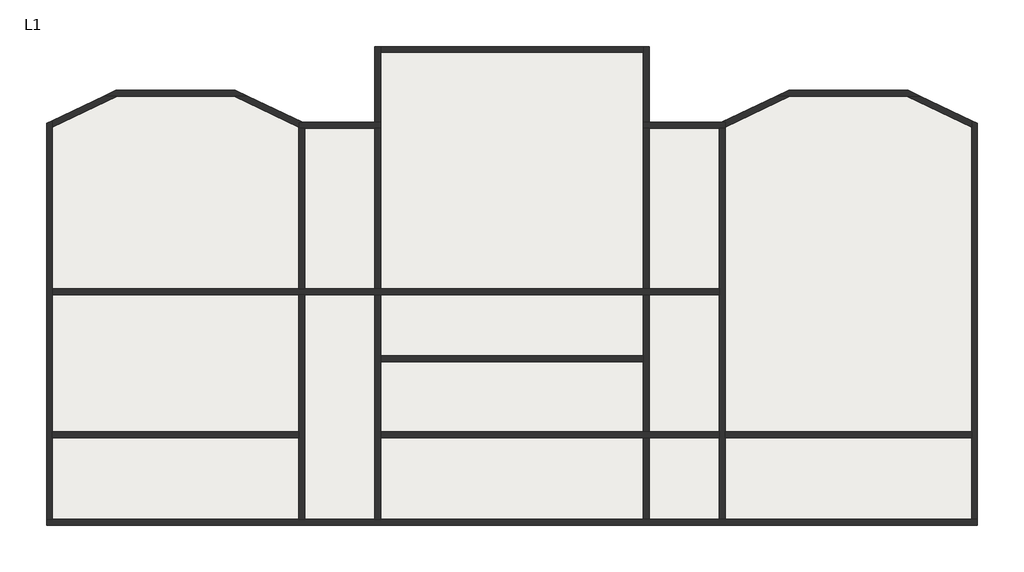
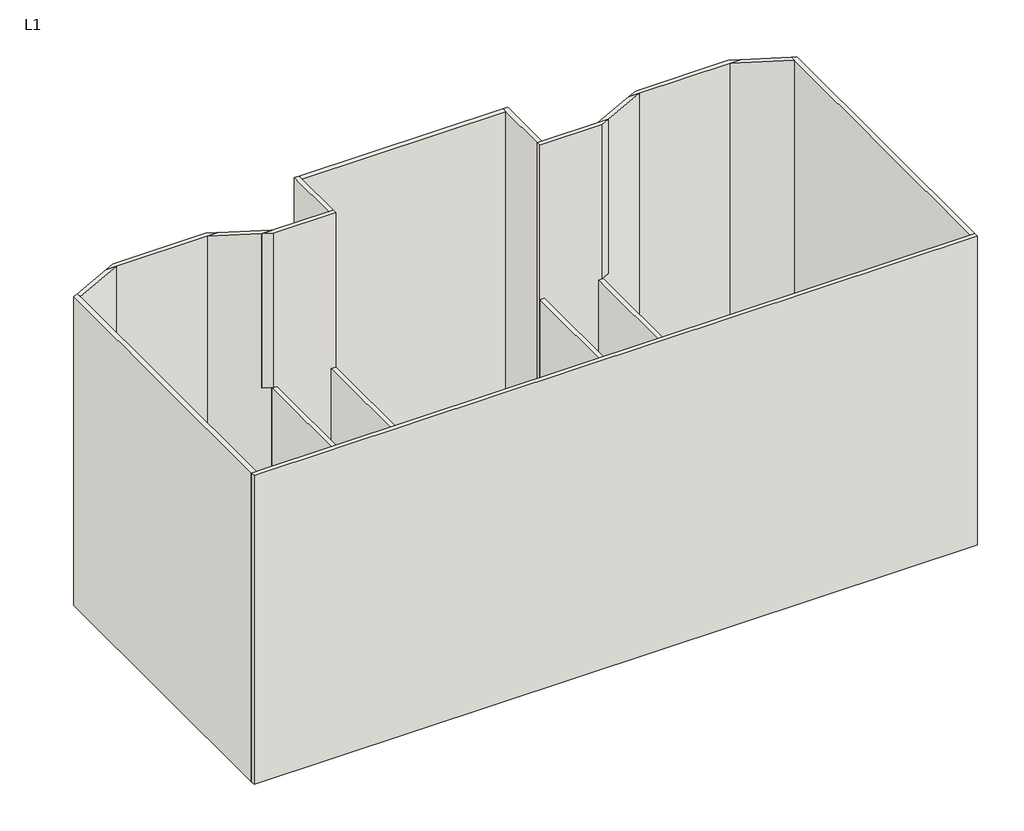
# One storey: 22 walls, 1 slab.
"""IFC4 building model written with IfcOpenShell, lengths in millimetres."""

import ifcopenshell
import ifcopenshell.guid

model = None  # the IFC model being written
_history = None  # IfcOwnerHistory: only IFC2X3 demands one
_inside = {}  # id of a spatial element -> (the spatial element, [elements in it])
_under = {}  # id of a project, library or spatial element -> (it, [spatial elements below it])
_declared = {}  # id of a project -> (the project, [libraries it declares])
_typed = {}  # id of a type object -> (the type object, [elements of that type])
_made_of = {}  # id of a material, layer set ... -> (it, [elements and type objects made of it])


def new_model(schema):
    """Start an empty IFC model of exactly this schema.

    Asked for "IFC4X3", IfcOpenShell would pick the latest addendum, in which some entities
    have other attributes; the version numbers below select the first issue.
    IFC2X3 requires an IfcOwnerHistory on every rooted entity: one is made here for all.
    """
    global model, _history
    if schema == "IFC4X3":
        model = ifcopenshell.file(schema_version=(4, 3, 0, 0))
    else:
        model = ifcopenshell.file(schema=schema)
    _inside.clear()
    _under.clear()
    _declared.clear()
    _typed.clear()
    _made_of.clear()
    _history = None
    if model.schema == "IFC2X3":
        org = make("IfcOrganization", Name="unknown")
        user = make(
            "IfcPersonAndOrganization",
            ThePerson=make("IfcPerson", FamilyName="unknown"),
            TheOrganization=org,
        )
        app = make(
            "IfcApplication",
            ApplicationDeveloper=org,
            Version="unknown",
            ApplicationFullName="unknown",
            ApplicationIdentifier="unknown",
        )
        _history = make(
            "IfcOwnerHistory",
            OwningUser=user,
            OwningApplication=app,
            ChangeAction="ADDED",
            CreationDate=0,
        )
    return model


def make(cls, **values):
    """One entity of the class cls with the attributes given. An attribute that is None is left unset."""
    return model.create_entity(
        cls, **{name: value for name, value in values.items() if value is not None}
    )


def rooted(cls, **values):
    """An entity with a GlobalId (a new one), such as an element, a storey or a relation."""
    return make(cls, GlobalId=ifcopenshell.guid.new(), OwnerHistory=_history, **values)


def si_unit(unit_type, name, prefix=None):
    """IfcSIUnit, for example si_unit("LENGTHUNIT", "METRE", prefix="MILLI")."""
    return make("IfcSIUnit", UnitType=unit_type, Prefix=prefix, Name=name)


def assignment(units):
    """IfcUnitAssignment: the units of a project."""
    return None if units is None else make("IfcUnitAssignment", Units=units)


def point(xyz):
    """IfcCartesianPoint."""
    return None if xyz is None else make("IfcCartesianPoint", Coordinates=xyz)


def direction(xyz):
    """IfcDirection."""
    return None if xyz is None else make("IfcDirection", DirectionRatios=xyz)


def frame(location, z_axis=None, x_axis=None):
    """IfcAxis2Placement3D, a coordinate frame: its origin and axes. An axis left out is left unset."""
    return make(
        "IfcAxis2Placement3D",
        Location=point(location),
        Axis=direction(z_axis),
        RefDirection=direction(x_axis),
    )


def origin():
    """The frame at (0, 0, 0) with its axes left unset."""
    return frame((0.0, 0.0, 0.0))


def origin_with_axes():
    """The frame at (0, 0, 0) with the z axis (0, 0, 1) and the x axis (1, 0, 0) written out."""
    return frame((0.0, 0.0, 0.0), z_axis=(0.0, 0.0, 1.0), x_axis=(1.0, 0.0, 0.0))


def place(relative_to, where):
    """IfcLocalPlacement: puts the frame where relative to a parent placement (None: the world)."""
    return make(
        "IfcLocalPlacement", PlacementRelTo=relative_to, RelativePlacement=where
    )


def context(
    kind, dimensions, precision=None, world=None, true_north=None, identifier=None
):
    """IfcGeometricRepresentationContext, for example the 3D "Model" context."""
    return make(
        "IfcGeometricRepresentationContext",
        ContextIdentifier=identifier,
        ContextType=kind,
        CoordinateSpaceDimension=dimensions,
        Precision=precision,
        WorldCoordinateSystem=world,
        TrueNorth=true_north,
    )


def project(units=None, contexts=None):
    """IfcProject with its units and contexts."""
    return rooted(
        "IfcProject",
        Name="project",
        RepresentationContexts=contexts,
        UnitsInContext=assignment(units),
    )


def spatial(cls, under=None, at=None, **own):
    """A site, building, storey or space (cls), placed at a placement, below another one or the project."""
    s = rooted(cls, ObjectPlacement=at, **own)
    if under is not None:
        _under.setdefault(under.id(), (under, []))[1].append(s)
    return s


def polyline(points):
    """IfcPolyline through the points."""
    return make("IfcPolyline", Points=[point(p) for p in points])


def outline(outer, holes=None, kind="AREA"):
    """IfcArbitraryClosedProfileDef: a profile drawn as a closed curve; with holes, ...WithVoids."""
    if holes is None:
        return make("IfcArbitraryClosedProfileDef", ProfileType=kind, OuterCurve=outer)
    return make(
        "IfcArbitraryProfileDefWithVoids",
        ProfileType=kind,
        OuterCurve=outer,
        InnerCurves=holes,
    )


def extrude(swept, where, along, depth):
    """IfcExtrudedAreaSolid: the profile swept, set in the frame where, extruded along a direction by depth."""
    return make(
        "IfcExtrudedAreaSolid",
        SweptArea=swept,
        Position=where,
        ExtrudedDirection=direction(along),
        Depth=depth,
    )


def faces_of(points, faces, orient=None, outer=None):
    """IfcFace entities. A face is a list of loops; a loop is a list of indices into points, from 0.

    orient and outer hold one flag for each loop. By default every Orientation is true, the
    first loop of a face is its IfcFaceOuterBound and the others are IfcFaceBound.
    """
    made = []
    for i, loops in enumerate(faces):
        bounds = []
        for j, loop in enumerate(loops):
            is_outer = j == 0 if outer is None else outer[i][j]
            bounds.append(
                make(
                    "IfcFaceOuterBound" if is_outer else "IfcFaceBound",
                    Bound=make("IfcPolyLoop", Polygon=[points[k] for k in loop]),
                    Orientation=True if orient is None else orient[i][j],
                )
            )
        made.append(make("IfcFace", Bounds=bounds))
    return made


def faceted_brep(points, faces, orient=None, outer=None, voids=None):
    """IfcFacetedBrep: a solid bounded by flat faces; with voids (closed shells), ...WithVoids."""
    shared = [point(p) for p in points]
    hull = make("IfcClosedShell", CfsFaces=faces_of(shared, faces, orient, outer))
    if voids is None:
        return make("IfcFacetedBrep", Outer=hull)
    return make(
        "IfcFacetedBrepWithVoids",
        Outer=hull,
        Voids=[
            make(cls, CfsFaces=faces_of(shared, fs, o, b)) for cls, fs, o, b in voids
        ],
    )


def shape(context_of_items, identifier, shape_type, items):
    """IfcShapeRepresentation: the items that make up one representation, for example the "Body"."""
    return make(
        "IfcShapeRepresentation",
        ContextOfItems=context_of_items,
        RepresentationIdentifier=identifier,
        RepresentationType=shape_type,
        Items=items,
    )


def made_of(thing, what):
    """Note that an element or type object is made of a material, layer set ...; save() writes the relation."""
    if what is not None:
        _made_of.setdefault(what.id(), (what, []))[1].append(thing)
    return thing


def element(
    cls,
    number,
    at=None,
    inside=None,
    cuts=None,
    type_object=None,
    material=None,
    context=None,
    identifier="Body",
    shape_type=None,
    held_by="IfcProductDefinitionShape",
    body=None,
    shapes=None,
    **own,
):
    """One element of the class cls, such as IfcWall. Its Tag is "e" and its number.

    at: its placement. inside: the storey or other place that contains it. cuts: it is an
    opening in that element (IfcRelVoidsElement). A single representation is given by context,
    identifier, shape_type and body (its items); several are given by shapes. held_by: the class
    of the entity that holds the representations. save() writes the other relations.
    """
    e = rooted(cls, Tag="e%d" % number, ObjectPlacement=at, **own)
    if body is not None:
        shapes = [shape(context, identifier, shape_type, body)]
    if shapes is not None:
        e.Representation = make(held_by, Representations=shapes)
    if inside is not None:
        _inside.setdefault(inside.id(), (inside, []))[1].append(e)
    if cuts is not None:
        rooted(
            "IfcRelVoidsElement", RelatingBuildingElement=cuts, RelatedOpeningElement=e
        )
    if type_object is not None:
        _typed.setdefault(type_object.id(), (type_object, []))[1].append(e)
    return made_of(e, material)


def aggregate(whole, parts):
    """IfcRelAggregates: a whole, such as a stair, and the parts it consists of."""
    return rooted("IfcRelAggregates", RelatingObject=whole, RelatedObjects=parts)


def save(model, path):
    """Write the relations noted so far, then the file.

    IfcRelAggregates (storeys below a building ...), IfcRelContainedInSpatialStructure (elements
    in a storey), IfcRelDefinesByType, IfcRelAssociatesMaterial and IfcRelDeclares: one each for
    every whole, place, type object, material and project.
    """
    for whole, parts in _under.values():
        aggregate(whole, parts)
    for where, things in _inside.values():
        rooted(
            "IfcRelContainedInSpatialStructure",
            RelatedElements=things,
            RelatingStructure=where,
        )
    for kind, things in _typed.values():
        rooted("IfcRelDefinesByType", RelatedObjects=things, RelatingType=kind)
    for what, things in _made_of.values():
        rooted("IfcRelAssociatesMaterial", RelatedObjects=things, RelatingMaterial=what)
    for by, libraries in _declared.values():
        rooted("IfcRelDeclares", RelatingContext=by, RelatedDefinitions=libraries)
    model.write(path)


model = new_model("IFC4")

# Units and contexts
model_context = context("Model", 3, world=origin())
ifc_project = project(units=[si_unit("LENGTHUNIT", "METRE", prefix="MILLI")], contexts=[model_context])

# Site, building, storey
site = spatial("IfcSite", under=ifc_project)
building = spatial("IfcBuilding", under=site)
storey = spatial("IfcBuildingStorey", under=building, Name="L1", Elevation=0.0)

# Slab
placement = place(None, origin())
element("IfcSlab", 1, ObjectType="Generic - 12\"", at=placement, inside=storey, context=model_context, shape_type="SweptSolid", body=[
    extrude(outline(polyline([(-6795.2529457, 14979.9250262), (-4760.8985742, 14979.9250262), (-3592.4985742, 14421.1250262), (-2209.3757599, 14421.1250262), (-2209.3757599, 15741.9250262), (2362.6242401, 15741.9250262), (2362.6242401, 14421.1250262), (3745.7470543, 14421.1250262), (4914.1470543, 14979.9250262), (6948.5014258, 14979.9250262), (8077.6242401, 14439.9097672), (8077.6242401, 7613.9250262), (-7924.3757599, 7613.9250262), (-7924.3757599, 14439.9097672), (-6795.2529457, 14979.9250262)])), origin_with_axes(), (0.0, 0.0, 1.0), 304.8),
])

# Walls
element("IfcWall", 2, ObjectType="Generic - 4\"", at=placement, inside=storey, context=model_context, shape_type="Brep", body=[
    faceted_brep([(-3631.7757599, 14421.1250262, 0.0), (-3530.1757599, 14421.1250262, 0.0), (-2310.9757599, 14421.1250262, 0.0), (-2209.3757599, 14421.1250262, 0.0), (-2209.3757599, 14421.1250262, 3657.6), (-2209.3757599, 14421.1250262, 7315.2), (-3592.4985742, 14421.1250262, 7315.2), (-3592.4985742, 14421.1250262, 3657.6), (-3631.7757599, 14421.1250262, 3657.6), (-3631.7757599, 14522.7250262, 0.0), (-3631.7757599, 14522.7250262, 3657.6), (-3804.9349378, 14522.7250262, 3657.6), (-3804.9349378, 14522.7250262, 7315.2), (-3569.4529457, 14522.7250262, 7315.2), (-2310.9757599, 14522.7250262, 7315.2), (-2209.3757599, 14522.7250262, 7315.2), (-2209.3757599, 14522.7250262, 0.0), (-2310.9757599, 14522.7250262, 0.0), (-3569.4529457, 14522.7250262, 0.0), (-3631.7757599, 14439.9097672, 0.0), (-3631.7757599, 14439.9097672, 3657.6)], [[[0, 1, 2, 3, 4, 5, 6, 7, 8]], [[9, 10, 11, 12, 13, 14, 15, 16, 17, 18]], [[3, 2, 1, 0, 19, 9, 18, 17, 16]], [[6, 5, 15, 14, 13, 12]], [[7, 20, 8]], [[0, 8, 20, 10, 9, 19]], [[7, 6, 12, 11, 20]], [[20, 11, 10]], [[3, 16, 15, 5, 4]]]),
])
element("IfcWall", 3, ObjectType="Generic - 4\"", at=placement, inside=storey, context=model_context, shape_type="Brep", body=[
    faceted_brep([(-4737.8529457, 15081.5250262, 0.0), (-6818.2985742, 15081.5250262, 0.0), (-6818.2985742, 15081.5250262, 7315.2), (-4737.8529457, 15081.5250262, 7315.2), (-4525.4165821, 14979.9250262, 0.0), (-4525.4165821, 14979.9250262, 7315.2), (-4760.8985742, 14979.9250262, 7315.2), (-6795.2529457, 14979.9250262, 7315.2), (-7030.7349378, 14979.9250262, 7315.2), (-7030.7349378, 14979.9250262, 0.0), (-6795.2529457, 14979.9250262, 0.0), (-4760.8985742, 14979.9250262, 0.0)], [[[0, 1, 2, 3]], [[4, 5, 6, 7, 8, 9, 10, 11]], [[1, 0, 4, 11, 10, 9]], [[3, 2, 8, 7, 6, 5]], [[0, 3, 5, 4]], [[2, 1, 9, 8]]]),
])
element("IfcWall", 4, ObjectType="Generic - 4\"", at=placement, inside=storey, context=model_context, shape_type="Brep", body=[
    faceted_brep([(-8025.9757599, 14503.9402852, 0.0), (-8025.9757599, 7613.9250262, 0.0), (-8025.9757599, 7613.9250262, 7315.2), (-8025.9757599, 14503.9402852, 7315.2), (-7924.3757599, 14552.5315895, 0.0), (-7924.3757599, 14552.5315895, 7315.2), (-7924.3757599, 14439.9097672, 7315.2), (-7924.3757599, 7613.9250262, 7315.2), (-7924.3757599, 7613.9250262, 3657.6), (-7924.3757599, 7613.9250262, 3352.8), (-7924.3757599, 7613.9250262, 0.0), (-7924.3757599, 9036.3250262, 0.0), (-7924.3757599, 9137.9250262, 0.0), (-7924.3757599, 11525.5250262, 0.0), (-7924.3757599, 11627.1250262, 0.0), (-7924.3757599, 14439.9097672, 0.0)], [[[0, 1, 2, 3]], [[4, 5, 6, 7, 8, 9, 10, 11, 12, 13, 14, 15]], [[1, 0, 4, 15, 14, 13, 12, 11, 10]], [[3, 2, 7, 6, 5]], [[2, 1, 10, 9, 8, 7]], [[0, 3, 5, 4]]]),
])
element("IfcWall", 5, ObjectType="Generic - 4\"", at=placement, inside=storey, context=model_context, shape_type="Brep", body=[
    faceted_brep([(-7924.3757599, 11525.5250262, 0.0), (-3631.7757599, 11525.5250262, 0.0), (-3530.1757599, 11525.5250262, 0.0), (-2310.9757599, 11525.5250262, 0.0), (-2209.3757599, 11525.5250262, 0.0), (2362.6242401, 11525.5250262, 0.0), (2464.2242401, 11525.5250262, 0.0), (3683.4242401, 11525.5250262, 0.0), (3683.4242401, 11525.5250262, 3352.8), (3683.4242401, 11525.5250262, 3657.6), (2464.2242401, 11525.5250262, 3657.6), (2362.6242401, 11525.5250262, 3657.6), (-2209.3757599, 11525.5250262, 3657.6), (-2310.9757599, 11525.5250262, 3657.6), (-3530.1757599, 11525.5250262, 3657.6), (-3530.1757599, 11525.5250262, 3352.8), (-3631.7757599, 11525.5250262, 3352.8), (-7924.3757599, 11525.5250262, 3352.8), (-7924.3757599, 11627.1250262, 0.0), (-7924.3757599, 11627.1250262, 3352.8), (-3530.1757599, 11627.1250262, 3352.8), (-3530.1757599, 11627.1250262, 3657.6), (-2310.9757599, 11627.1250262, 3657.6), (-2209.3757599, 11627.1250262, 3657.6), (2362.6242401, 11627.1250262, 3657.6), (2464.2242401, 11627.1250262, 3657.6), (3683.4242401, 11627.1250262, 3657.6), (3683.4242401, 11627.1250262, 0.0), (2464.2242401, 11627.1250262, 0.0), (2362.6242401, 11627.1250262, 0.0), (-2209.3757599, 11627.1250262, 0.0), (-2310.9757599, 11627.1250262, 0.0), (-3530.1757599, 11627.1250262, 0.0), (-3631.7757599, 11627.1250262, 0.0)], [[[0, 1, 2, 3, 4, 5, 6, 7, 8, 9, 10, 11, 12, 13, 14, 15, 16, 17]], [[18, 19, 20, 21, 22, 23, 24, 25, 26, 27, 28, 29, 30, 31, 32, 33]], [[7, 6, 5, 4, 3, 2, 1, 0, 18, 33, 32, 31, 30, 29, 28, 27]], [[0, 17, 19, 18]], [[9, 8, 7, 27, 26]], [[14, 13, 12, 11, 10, 9, 26, 25, 24, 23, 22, 21]], [[14, 21, 20, 15]], [[17, 16, 15, 20, 19]]]),
])
element("IfcWall", 6, ObjectType="Generic - 4\"", at=placement, inside=storey, context=model_context, shape_type="SweptSolid", body=[
    extrude(outline(polyline([(-3631.7757599, 9036.3250262), (-7924.3757599, 9036.3250262), (-7924.3757599, 9137.9250262), (-3631.7757599, 9137.9250262), (-3631.7757599, 9036.3250262)])), origin_with_axes(), (0.0, 0.0, 1.0), 3352.8),
])
element("IfcWall", 7, ObjectType="Generic - 4\"", at=placement, inside=storey, context=model_context, shape_type="Brep", body=[
    faceted_brep([(-3631.7757599, 14421.1250262, 3657.6), (-3631.7757599, 14421.1250262, 0.0), (-3631.7757599, 11627.1250262, 0.0), (-3631.7757599, 11627.1250262, 3657.6), (-3530.1757599, 14421.1250262, 0.0), (-3530.1757599, 14421.1250262, 3657.6), (-3530.1757599, 11627.1250262, 3657.6), (-3530.1757599, 11627.1250262, 0.0), (-3592.4985742, 14421.1250262, 3657.6)], [[[0, 1, 2, 3]], [[4, 5, 6, 7]], [[1, 4, 7, 2]], [[1, 0, 8, 5, 4]], [[5, 8, 0, 3, 6]], [[6, 3, 2, 7]]]),
    faceted_brep([(-3631.7757599, 7613.9250262, 0.0), (-3631.7757599, 7613.9250262, 3352.8), (-3631.7757599, 9036.3250262, 3352.8), (-3631.7757599, 9137.9250262, 3352.8), (-3631.7757599, 11525.5250262, 3352.8), (-3631.7757599, 11525.5250262, 0.0), (-3631.7757599, 9137.9250262, 0.0), (-3631.7757599, 9036.3250262, 0.0), (-3530.1757599, 7613.9250262, 3352.8), (-3530.1757599, 7613.9250262, 0.0), (-3530.1757599, 11525.5250262, 0.0), (-3530.1757599, 11525.5250262, 3352.8), (-3530.1757599, 10458.7250262, 3352.8)], [[[0, 1, 2, 3, 4, 5, 6, 7]], [[8, 9, 10, 11, 12]], [[9, 0, 7, 6, 5, 10]], [[5, 4, 11, 10]], [[1, 0, 9, 8]], [[1, 8, 12, 11, 4, 3, 2]]]),
])
element("IfcWall", 8, ObjectType="Generic - 4\"", at=placement, inside=storey, context=model_context, shape_type="Brep", body=[
    faceted_brep([(-4760.8985742, 14979.9250262, 0.0), (-3631.7757599, 14439.9097672, 0.0), (-3631.7757599, 14439.9097672, 3657.6), (-3804.9349378, 14522.7250262, 3657.6), (-3804.9349378, 14522.7250262, 7315.2), (-4760.8985742, 14979.9250262, 7315.2), (-4525.4165821, 14979.9250262, 0.0), (-4525.4165821, 14979.9250262, 7315.2), (-3569.4529457, 14522.7250262, 7315.2), (-3569.4529457, 14522.7250262, 3657.6), (-3569.4529457, 14522.7250262, 0.0), (-3631.7757599, 14522.7250262, 0.0), (-3631.7757599, 14522.7250262, 3657.6)], [[[0, 1, 2, 3, 4, 5]], [[6, 7, 8, 9, 10]], [[1, 0, 6, 10, 11]], [[5, 4, 8, 7]], [[0, 5, 7, 6]], [[11, 10, 9, 12]], [[12, 3, 2]], [[2, 1, 11, 12]], [[4, 3, 12, 9, 8]]]),
])
element("IfcWall", 9, ObjectType="Generic - 4\"", at=placement, inside=storey, context=model_context, shape_type="SweptSolid", body=[
    extrude(outline(polyline([(-6795.2529457, 14979.9250262), (-7924.3757599, 14439.9097672), (-7924.3757599, 14552.5315895), (-7030.7349378, 14979.9250262), (-6795.2529457, 14979.9250262)])), origin_with_axes(), (0.0, 0.0, 1.0), 7315.2),
])
element("IfcWall", 10, ObjectType="Generic - 4\"", at=placement, inside=storey, context=model_context, shape_type="Brep", body=[
    faceted_brep([(-2310.9757599, 15843.5250262, 0.0), (-2310.9757599, 14522.7250262, 0.0), (-2310.9757599, 14522.7250262, 7315.2), (-2310.9757599, 15843.5250262, 7315.2), (-2209.3757599, 15843.5250262, 0.0), (-2209.3757599, 15843.5250262, 7315.2), (-2209.3757599, 15741.9250262, 7315.2), (-2209.3757599, 14522.7250262, 7315.2), (-2209.3757599, 14522.7250262, 0.0), (-2209.3757599, 15741.9250262, 0.0)], [[[0, 1, 2, 3]], [[4, 5, 6, 7, 8, 9]], [[1, 0, 4, 9, 8]], [[3, 2, 7, 6, 5]], [[0, 3, 5, 4]], [[1, 8, 7, 2]]]),
])
element("IfcWall", 11, ObjectType="Generic - 4\"", at=placement, inside=storey, context=model_context, shape_type="SweptSolid", body=[
    extrude(outline(polyline([(2362.6242401, 15741.9250262), (-2209.3757599, 15741.9250262), (-2209.3757599, 15843.5250262), (2362.6242401, 15843.5250262), (2362.6242401, 15741.9250262)])), origin_with_axes(), (0.0, 0.0, 1.0), 7315.2),
])
element("IfcWall", 12, ObjectType="Generic - 4\"", at=placement, inside=storey, context=model_context, shape_type="Brep", body=[
    faceted_brep([(3785.0242401, 14522.7250262, 0.0), (3722.7014258, 14522.7250262, 0.0), (2464.2242401, 14522.7250262, 0.0), (2362.6242401, 14522.7250262, 0.0), (2362.6242401, 14522.7250262, 7315.2), (2464.2242401, 14522.7250262, 7315.2), (3722.7014258, 14522.7250262, 7315.2), (3958.1834179, 14522.7250262, 7315.2), (3958.1834179, 14522.7250262, 3657.6), (3785.0242401, 14522.7250262, 3657.6), (3785.0242401, 14421.1250262, 0.0), (3785.0242401, 14421.1250262, 3657.6), (3745.7470543, 14421.1250262, 3657.6), (3745.7470543, 14421.1250262, 7315.2), (2362.6242401, 14421.1250262, 7315.2), (2362.6242401, 14421.1250262, 3657.6), (2362.6242401, 14421.1250262, 0.0), (2464.2242401, 14421.1250262, 0.0), (3683.4242401, 14421.1250262, 0.0), (3785.0242401, 14439.9097672, 0.0), (3785.0242401, 14439.9097672, 3657.6)], [[[0, 1, 2, 3, 4, 5, 6, 7, 8, 9]], [[10, 11, 12, 13, 14, 15, 16, 17, 18]], [[3, 2, 1, 0, 19, 10, 18, 17, 16]], [[7, 6, 5, 4, 14, 13]], [[8, 20, 9]], [[0, 9, 20, 11, 10, 19]], [[8, 7, 13, 12, 20]], [[20, 12, 11]], [[3, 16, 15, 14, 4]]]),
])
element("IfcWall", 13, ObjectType="Generic - 4\"", at=placement, inside=storey, context=model_context, shape_type="Brep", body=[
    faceted_brep([(4678.6650622, 14979.9250262, 0.0), (4914.1470543, 14979.9250262, 0.0), (6948.5014258, 14979.9250262, 0.0), (7183.9834179, 14979.9250262, 0.0), (7183.9834179, 14979.9250262, 7315.2), (6948.5014258, 14979.9250262, 7315.2), (4914.1470543, 14979.9250262, 7315.2), (4678.6650622, 14979.9250262, 7315.2), (4891.1014258, 15081.5250262, 0.0), (4891.1014258, 15081.5250262, 7315.2), (6971.5470543, 15081.5250262, 7315.2), (6971.5470543, 15081.5250262, 0.0)], [[[0, 1, 2, 3, 4, 5, 6, 7]], [[8, 9, 10, 11]], [[3, 2, 1, 0, 8, 11]], [[7, 6, 5, 4, 10, 9]], [[0, 7, 9, 8]], [[4, 3, 11, 10]]]),
])
element("IfcWall", 14, ObjectType="Generic - 4\"", at=placement, inside=storey, context=model_context, shape_type="Brep", body=[
    faceted_brep([(8077.6242401, 14552.5315895, 0.0), (8077.6242401, 14439.9097672, 0.0), (8077.6242401, 9137.9250262, 0.0), (8077.6242401, 9036.3250262, 0.0), (8077.6242401, 7613.9250262, 0.0), (8077.6242401, 7613.9250262, 3352.8), (8077.6242401, 7613.9250262, 3657.6), (8077.6242401, 7613.9250262, 7315.2), (8077.6242401, 14439.9097672, 7315.2), (8077.6242401, 14552.5315895, 7315.2), (8179.2242401, 14503.9402852, 0.0), (8179.2242401, 14503.9402852, 7315.2), (8179.2242401, 7613.9250262, 7315.2), (8179.2242401, 7613.9250262, 0.0)], [[[0, 1, 2, 3, 4, 5, 6, 7, 8, 9]], [[10, 11, 12, 13]], [[4, 3, 2, 1, 0, 10, 13]], [[9, 8, 7, 12, 11]], [[7, 6, 5, 4, 13, 12]], [[0, 9, 11, 10]]]),
])
element("IfcWall", 15, ObjectType="Generic - 4\"", at=placement, inside=storey, context=model_context, shape_type="Brep", body=[
    faceted_brep([(3683.4242401, 14421.1250262, 0.0), (3683.4242401, 11627.1250262, 0.0), (3683.4242401, 11525.5250262, 0.0), (3683.4242401, 9137.9250262, 0.0), (3683.4242401, 9036.3250262, 0.0), (3683.4242401, 7613.9250262, 0.0), (3683.4242401, 7613.9250262, 3352.8), (3683.4242401, 9036.3250262, 3352.8), (3683.4242401, 9137.9250262, 3352.8), (3683.4242401, 10458.7250262, 3352.8), (3683.4242401, 11525.5250262, 3352.8), (3683.4242401, 11525.5250262, 3657.6), (3683.4242401, 11627.1250262, 3657.6), (3683.4242401, 14421.1250262, 3657.6), (3785.0242401, 14421.1250262, 0.0), (3785.0242401, 14421.1250262, 3657.6), (3785.0242401, 11525.5250262, 3657.6), (3785.0242401, 11525.5250262, 3352.8), (3785.0242401, 9137.9250262, 3352.8), (3785.0242401, 9036.3250262, 3352.8), (3785.0242401, 7613.9250262, 3352.8), (3785.0242401, 7613.9250262, 0.0), (3785.0242401, 9036.3250262, 0.0), (3785.0242401, 9137.9250262, 0.0), (3745.7470543, 14421.1250262, 3657.6)], [[[0, 1, 2, 3, 4, 5, 6, 7, 8, 9, 10, 11, 12, 13]], [[14, 15, 16, 17, 18, 19, 20, 21, 22, 23]], [[5, 4, 3, 2, 1, 0, 14, 23, 22, 21]], [[0, 13, 24, 15, 14]], [[6, 5, 21, 20]], [[13, 12, 11, 16, 15, 24]], [[16, 11, 10, 17]], [[10, 9, 8, 7, 6, 20, 19, 18, 17]]]),
])
element("IfcWall", 16, ObjectType="Generic - 4\"", at=placement, inside=storey, context=model_context, shape_type="Brep", body=[
    faceted_brep([(-8025.9757599, 7512.3250262, 0.0), (8179.2242401, 7512.3250262, 0.0), (8179.2242401, 7512.3250262, 7315.2), (-8025.9757599, 7512.3250262, 7315.2), (-8025.9757599, 7613.9250262, 0.0), (-8025.9757599, 7613.9250262, 7315.2), (-7924.3757599, 7613.9250262, 7315.2), (8077.6242401, 7613.9250262, 7315.2), (8179.2242401, 7613.9250262, 7315.2), (8179.2242401, 7613.9250262, 0.0), (8077.6242401, 7613.9250262, 0.0), (3785.0242401, 7613.9250262, 0.0), (3683.4242401, 7613.9250262, 0.0), (2464.2242401, 7613.9250262, 0.0), (2362.6242401, 7613.9250262, 0.0), (-2209.3757599, 7613.9250262, 0.0), (-2310.9757599, 7613.9250262, 0.0), (-3530.1757599, 7613.9250262, 0.0), (-3631.7757599, 7613.9250262, 0.0), (-7924.3757599, 7613.9250262, 0.0)], [[[0, 1, 2, 3]], [[4, 5, 6, 7, 8, 9, 10, 11, 12, 13, 14, 15, 16, 17, 18, 19]], [[1, 0, 4, 19, 18, 17, 16, 15, 14, 13, 12, 11, 10, 9]], [[3, 2, 8, 7, 6, 5]], [[2, 1, 9, 8]], [[0, 3, 5, 4]]]),
])
element("IfcWall", 17, ObjectType="Generic - 4\"", at=placement, inside=storey, context=model_context, shape_type="Brep", body=[
    faceted_brep([(4678.6650622, 14979.9250262, 0.0), (3722.7014258, 14522.7250262, 0.0), (3722.7014258, 14522.7250262, 3657.6), (3722.7014258, 14522.7250262, 7315.2), (4678.6650622, 14979.9250262, 7315.2), (4914.1470543, 14979.9250262, 0.0), (4914.1470543, 14979.9250262, 7315.2), (3958.1834179, 14522.7250262, 7315.2), (3958.1834179, 14522.7250262, 3657.6), (3785.0242401, 14439.9097672, 3657.6), (3785.0242401, 14439.9097672, 0.0), (3785.0242401, 14522.7250262, 0.0), (3785.0242401, 14522.7250262, 3657.6)], [[[0, 1, 2, 3, 4]], [[5, 6, 7, 8, 9, 10]], [[1, 0, 5, 10, 11]], [[4, 3, 7, 6]], [[0, 4, 6, 5]], [[11, 10, 9, 12]], [[8, 12, 9]], [[2, 1, 11, 12]], [[3, 2, 12, 8, 7]]]),
])
element("IfcWall", 18, ObjectType="Generic - 4\"", at=placement, inside=storey, context=model_context, shape_type="SweptSolid", body=[
    extrude(outline(polyline([(7183.9834179, 14979.9250262), (8077.6242401, 14552.5315895), (8077.6242401, 14439.9097672), (6948.5014258, 14979.9250262), (7183.9834179, 14979.9250262)])), origin_with_axes(), (0.0, 0.0, 1.0), 7315.2),
])
element("IfcWall", 19, ObjectType="Generic - 4\"", at=placement, inside=storey, context=model_context, shape_type="Brep", body=[
    faceted_brep([(2362.6242401, 15843.5250262, 0.0), (2362.6242401, 15741.9250262, 0.0), (2362.6242401, 14522.7250262, 0.0), (2362.6242401, 14522.7250262, 7315.2), (2362.6242401, 15741.9250262, 7315.2), (2362.6242401, 15843.5250262, 7315.2), (2464.2242401, 15843.5250262, 0.0), (2464.2242401, 15843.5250262, 7315.2), (2464.2242401, 14522.7250262, 7315.2), (2464.2242401, 14522.7250262, 0.0)], [[[0, 1, 2, 3, 4, 5]], [[6, 7, 8, 9]], [[2, 1, 0, 6, 9]], [[5, 4, 3, 8, 7]], [[0, 5, 7, 6]], [[2, 9, 8, 3]]]),
])
element("IfcWall", 20, ObjectType="Generic - 4\"", at=placement, inside=storey, context=model_context, shape_type="SweptSolid", body=[
    extrude(outline(polyline([(2362.6242401, 10357.1250262), (-2209.3757599, 10357.1250262), (-2209.3757599, 10458.7250262), (2362.6242401, 10458.7250262), (2362.6242401, 10357.1250262)])), origin_with_axes(), (0.0, 0.0, 1.0), 3352.8),
])
element("IfcWall", 21, ObjectType="Generic - 4\"", at=placement, inside=storey, context=model_context, shape_type="Brep", body=[
    faceted_brep([(8077.6242401, 9036.3250262, 0.0), (8077.6242401, 9036.3250262, 3352.8), (3785.0242401, 9036.3250262, 3352.8), (3785.0242401, 9036.3250262, 0.0), (8077.6242401, 9137.9250262, 3352.8), (8077.6242401, 9137.9250262, 0.0), (3785.0242401, 9137.9250262, 0.0), (3785.0242401, 9137.9250262, 3352.8)], [[[0, 1, 2, 3]], [[4, 5, 6, 7]], [[5, 0, 3, 6]], [[1, 0, 5, 4]], [[3, 2, 7, 6]], [[1, 4, 7, 2]]]),
    faceted_brep([(-2209.3757599, 9036.3250262, 3352.8), (-2209.3757599, 9036.3250262, 0.0), (2362.6242401, 9036.3250262, 0.0), (2464.2242401, 9036.3250262, 0.0), (3683.4242401, 9036.3250262, 0.0), (3683.4242401, 9036.3250262, 3352.8), (2464.2242401, 9036.3250262, 3352.8), (2362.6242401, 9036.3250262, 3352.8), (-2209.3757599, 9137.9250262, 0.0), (-2209.3757599, 9137.9250262, 3352.8), (2362.6242401, 9137.9250262, 3352.8), (2464.2242401, 9137.9250262, 3352.8), (3683.4242401, 9137.9250262, 3352.8), (3683.4242401, 9137.9250262, 0.0), (2464.2242401, 9137.9250262, 0.0), (2362.6242401, 9137.9250262, 0.0)], [[[0, 1, 2, 3, 4, 5, 6, 7]], [[8, 9, 10, 11, 12, 13, 14, 15]], [[1, 8, 15, 14, 13, 4, 3, 2]], [[5, 4, 13, 12]], [[1, 0, 9, 8]], [[9, 0, 7, 6, 5, 12, 11, 10]]]),
])
element("IfcWall", 22, ObjectType="Generic - 4\"", at=placement, inside=storey, context=model_context, shape_type="Brep", body=[
    faceted_brep([(2464.2242401, 7613.9250262, 3352.8), (2464.2242401, 7613.9250262, 0.0), (2464.2242401, 9036.3250262, 0.0), (2464.2242401, 9036.3250262, 3352.8), (2362.6242401, 7613.9250262, 0.0), (2362.6242401, 7613.9250262, 3352.8), (2362.6242401, 9036.3250262, 3352.8), (2362.6242401, 9036.3250262, 0.0)], [[[0, 1, 2, 3]], [[4, 5, 6, 7]], [[1, 4, 7, 2]], [[1, 0, 5, 4]], [[3, 2, 7, 6]], [[5, 0, 3, 6]]]),
    faceted_brep([(2464.2242401, 14421.1250262, 0.0), (2464.2242401, 14421.1250262, 3657.6), (2464.2242401, 11627.1250262, 3657.6), (2464.2242401, 11627.1250262, 0.0), (2362.6242401, 14421.1250262, 3657.6), (2362.6242401, 14421.1250262, 0.0), (2362.6242401, 11627.1250262, 0.0), (2362.6242401, 11627.1250262, 3657.6)], [[[0, 1, 2, 3]], [[4, 5, 6, 7]], [[5, 0, 3, 6]], [[1, 0, 5, 4]], [[3, 2, 7, 6]], [[1, 4, 7, 2]]]),
    faceted_brep([(2464.2242401, 11525.5250262, 0.0), (2464.2242401, 11525.5250262, 3657.6), (2464.2242401, 10458.7250262, 3657.6), (2464.2242401, 10458.7250262, 3352.8), (2464.2242401, 9137.9250262, 3352.8), (2464.2242401, 9137.9250262, 0.0), (2362.6242401, 11525.5250262, 3657.6), (2362.6242401, 11525.5250262, 0.0), (2362.6242401, 10458.7250262, 0.0), (2362.6242401, 10357.1250262, 0.0), (2362.6242401, 9137.9250262, 0.0), (2362.6242401, 9137.9250262, 3352.8), (2362.6242401, 10357.1250262, 3352.8), (2362.6242401, 10458.7250262, 3352.8), (2362.6242401, 10458.7250262, 3657.6)], [[[0, 1, 2, 3, 4, 5]], [[6, 7, 8, 9, 10, 11, 12, 13, 14]], [[7, 0, 5, 10, 9, 8]], [[1, 0, 7, 6]], [[5, 4, 11, 10]], [[14, 2, 1, 6]], [[2, 14, 13, 3]], [[3, 13, 12, 11, 4]]]),
])
element("IfcWall", 23, ObjectType="Generic - 4\"", at=placement, inside=storey, context=model_context, shape_type="Brep", body=[
    faceted_brep([(-2209.3757599, 7613.9250262, 3352.8), (-2209.3757599, 7613.9250262, 0.0), (-2209.3757599, 9036.3250262, 0.0), (-2209.3757599, 9137.9250262, 0.0), (-2209.3757599, 10357.1250262, 0.0), (-2209.3757599, 10458.7250262, 0.0), (-2209.3757599, 11525.5250262, 0.0), (-2209.3757599, 11525.5250262, 3657.6), (-2209.3757599, 10458.7250262, 3657.6), (-2209.3757599, 10458.7250262, 3352.8), (-2209.3757599, 10357.1250262, 3352.8), (-2209.3757599, 9137.9250262, 3352.8), (-2209.3757599, 9036.3250262, 3352.8), (-2310.9757599, 7613.9250262, 0.0), (-2310.9757599, 7613.9250262, 3352.8), (-2310.9757599, 10458.7250262, 3352.8), (-2310.9757599, 10458.7250262, 3657.6), (-2310.9757599, 11525.5250262, 3657.6), (-2310.9757599, 11525.5250262, 0.0)], [[[0, 1, 2, 3, 4, 5, 6, 7, 8, 9, 10, 11, 12]], [[13, 14, 15, 16, 17, 18]], [[1, 13, 18, 6, 5, 4, 3, 2]], [[1, 0, 14, 13]], [[7, 6, 18, 17]], [[16, 8, 7, 17]], [[8, 16, 15, 9]], [[14, 0, 12, 11, 10, 9, 15]]]),
    faceted_brep([(-2209.3757599, 14421.1250262, 0.0), (-2209.3757599, 14421.1250262, 3657.6), (-2209.3757599, 11627.1250262, 3657.6), (-2209.3757599, 11627.1250262, 0.0), (-2310.9757599, 14421.1250262, 3657.6), (-2310.9757599, 14421.1250262, 0.0), (-2310.9757599, 11627.1250262, 0.0), (-2310.9757599, 11627.1250262, 3657.6)], [[[0, 1, 2, 3]], [[4, 5, 6, 7]], [[5, 0, 3, 6]], [[1, 0, 5, 4]], [[3, 2, 7, 6]], [[1, 4, 7, 2]]]),
])

save(model, "model.ifc")

# Revit data of these elements
# Project information
#   Organization Name = "Organization Name"
#   Organization Description = "Organization Description"
#   Building Name = "Building Name"
#   Project Issue Date = "Issue Date"
#   Project Status = "Project Status"
#   Client Name = "Client Name"
#   Project Address = "Enter address here\nAddress Line 2"
#   Project Name = "Project Name"
#   Project Number = "Project Number"
# Type "Generic - 12\""
#   Description = "Generic Floor (Material By Category), 12\" thick"
#   Type Mark = "G01"
#   Function = 0
#   Layers, outside or top first: 1' - 0" no material (function 1)
# Type "Generic - 4\""
#   Description = "Generic Wall (Material By Category), 4\" thick"
#   Type Mark = "G01"
#   Layers, outside or top first: 0' - 4" no material (function 1)
# Element 1 (IfcSlab, "Generic - 12\"")
#   built-in parameter 1001955 = 3.14159 (stored number, unit not read)
#   Height Offset From Level = 1' - 0"
#   Phase Created = New Construction
#   Materials on its faces: "Default Floor"
# Elements 2, 3, 4, 8, 9, 10, 11, 12, 13, 14, 16, 17, 18, 19 (IfcWall, "Generic - 4\"")
#   Top Offset = 0' - 0"
#   Base Offset = 0' - 0"
#   wall height = 24' - 0"
#   Phase Created = New Construction
#   Base Constraint = L1
#   Top Constraint = L3
#   Materials on its faces: "Default Wall"
# Elements 5, 6, 7, 15, 20, 21, 22, 23 (IfcWall, "Generic - 4\"")
#   Top Offset = 0' - 0"
#   Base Offset = 0' - 0"
#   wall height = 12' - 0"
#   Phase Created = New Construction
#   Base Constraint = L1
#   Top Constraint = L2
#   Materials on its faces: "Default Wall"
# Materials
#   "Default Floor": class "Miscellaneous", colour RGB 128 128 128, transparency 0, Cost = 0
#   "Default Wall": class "Miscellaneous", colour RGB 192 192 192, transparency 0, Cost = 0
